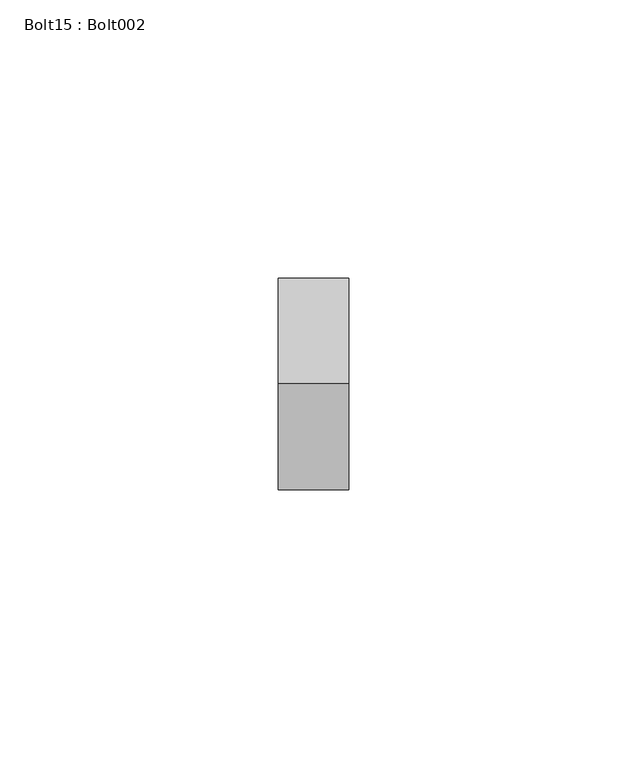
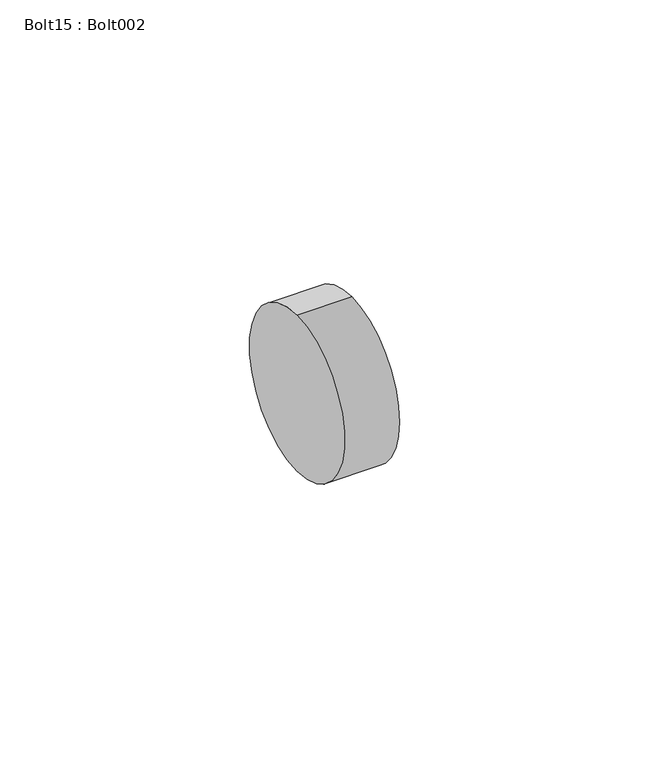
"""IFC4 building model written with IfcOpenShell, lengths in millimetres: proxy geometry, Bolt15 : Bolt002."""

import ifcopenshell
import ifcopenshell.guid

model = None  # the IFC model being written
_history = None  # IfcOwnerHistory: only IFC2X3 demands one
_inside = {}  # id of a spatial element -> (the spatial element, [elements in it])
_under = {}  # id of a project, library or spatial element -> (it, [spatial elements below it])
_declared = {}  # id of a project -> (the project, [libraries it declares])
_typed = {}  # id of a type object -> (the type object, [elements of that type])
_made_of = {}  # id of a material, layer set ... -> (it, [elements and type objects made of it])


def new_model(schema):
    """Start an empty IFC model of exactly this schema.

    Asked for "IFC4X3", IfcOpenShell would pick the latest addendum, in which some entities
    have other attributes; the version numbers below select the first issue.
    IFC2X3 requires an IfcOwnerHistory on every rooted entity: one is made here for all.
    """
    global model, _history
    if schema == "IFC4X3":
        model = ifcopenshell.file(schema_version=(4, 3, 0, 0))
    else:
        model = ifcopenshell.file(schema=schema)
    _inside.clear()
    _under.clear()
    _declared.clear()
    _typed.clear()
    _made_of.clear()
    _history = None
    if model.schema == "IFC2X3":
        org = make("IfcOrganization", Name="unknown")
        user = make(
            "IfcPersonAndOrganization",
            ThePerson=make("IfcPerson", FamilyName="unknown"),
            TheOrganization=org,
        )
        app = make(
            "IfcApplication",
            ApplicationDeveloper=org,
            Version="unknown",
            ApplicationFullName="unknown",
            ApplicationIdentifier="unknown",
        )
        _history = make(
            "IfcOwnerHistory",
            OwningUser=user,
            OwningApplication=app,
            ChangeAction="ADDED",
            CreationDate=0,
        )
    return model


def make(cls, **values):
    """One entity of the class cls with the attributes given. An attribute that is None is left unset."""
    return model.create_entity(
        cls, **{name: value for name, value in values.items() if value is not None}
    )


def rooted(cls, **values):
    """An entity with a GlobalId (a new one), such as an element, a storey or a relation."""
    return make(cls, GlobalId=ifcopenshell.guid.new(), OwnerHistory=_history, **values)


def si_unit(unit_type, name, prefix=None):
    """IfcSIUnit, for example si_unit("LENGTHUNIT", "METRE", prefix="MILLI")."""
    return make("IfcSIUnit", UnitType=unit_type, Prefix=prefix, Name=name)


def assignment(units):
    """IfcUnitAssignment: the units of a project."""
    return None if units is None else make("IfcUnitAssignment", Units=units)


def point(xyz):
    """IfcCartesianPoint."""
    return None if xyz is None else make("IfcCartesianPoint", Coordinates=xyz)


def direction(xyz):
    """IfcDirection."""
    return None if xyz is None else make("IfcDirection", DirectionRatios=xyz)


def frame(location, z_axis=None, x_axis=None):
    """IfcAxis2Placement3D, a coordinate frame: its origin and axes. An axis left out is left unset."""
    return make(
        "IfcAxis2Placement3D",
        Location=point(location),
        Axis=direction(z_axis),
        RefDirection=direction(x_axis),
    )


def frame_2d(location, x_axis=None):
    """IfcAxis2Placement2D, a coordinate frame in the plane: its origin and x axis."""
    return make(
        "IfcAxis2Placement2D", Location=point(location), RefDirection=direction(x_axis)
    )


def origin():
    """The frame at (0, 0, 0) with its axes left unset."""
    return frame((0.0, 0.0, 0.0))


def place(relative_to, where):
    """IfcLocalPlacement: puts the frame where relative to a parent placement (None: the world)."""
    return make(
        "IfcLocalPlacement", PlacementRelTo=relative_to, RelativePlacement=where
    )


def context(
    kind, dimensions, precision=None, world=None, true_north=None, identifier=None
):
    """IfcGeometricRepresentationContext, for example the 3D "Model" context."""
    return make(
        "IfcGeometricRepresentationContext",
        ContextIdentifier=identifier,
        ContextType=kind,
        CoordinateSpaceDimension=dimensions,
        Precision=precision,
        WorldCoordinateSystem=world,
        TrueNorth=true_north,
    )


def project(units=None, contexts=None):
    """IfcProject with its units and contexts."""
    return rooted(
        "IfcProject",
        Name="project",
        RepresentationContexts=contexts,
        UnitsInContext=assignment(units),
    )


def spatial(cls, under=None, at=None, **own):
    """A site, building, storey or space (cls), placed at a placement, below another one or the project."""
    s = rooted(cls, ObjectPlacement=at, **own)
    if under is not None:
        _under.setdefault(under.id(), (under, []))[1].append(s)
    return s


def circle_curve(where, radius):
    """IfcCircle in the frame where."""
    return make("IfcCircle", Position=where, Radius=radius)


def trimmed(basis, trim1, trim2, sense, master):
    """IfcTrimmedCurve: the piece of a basis curve between two trims."""
    return make(
        "IfcTrimmedCurve",
        BasisCurve=basis,
        Trim1=trim1,
        Trim2=trim2,
        SenseAgreement=sense,
        MasterRepresentation=master,
    )


def segment(curve, same_sense, transition):
    """IfcCompositeCurveSegment."""
    return make(
        "IfcCompositeCurveSegment",
        Transition=transition,
        SameSense=same_sense,
        ParentCurve=curve,
    )


def composite_curve(segments, self_intersect=None):
    """IfcCompositeCurve: segments joined end to end."""
    return make("IfcCompositeCurve", Segments=segments, SelfIntersect=self_intersect)


def outline(outer, holes=None, kind="AREA"):
    """IfcArbitraryClosedProfileDef: a profile drawn as a closed curve; with holes, ...WithVoids."""
    if holes is None:
        return make("IfcArbitraryClosedProfileDef", ProfileType=kind, OuterCurve=outer)
    return make(
        "IfcArbitraryProfileDefWithVoids",
        ProfileType=kind,
        OuterCurve=outer,
        InnerCurves=holes,
    )


def extrude(swept, where, along, depth):
    """IfcExtrudedAreaSolid: the profile swept, set in the frame where, extruded along a direction by depth."""
    return make(
        "IfcExtrudedAreaSolid",
        SweptArea=swept,
        Position=where,
        ExtrudedDirection=direction(along),
        Depth=depth,
    )


def shape(context_of_items, identifier, shape_type, items):
    """IfcShapeRepresentation: the items that make up one representation, for example the "Body"."""
    return make(
        "IfcShapeRepresentation",
        ContextOfItems=context_of_items,
        RepresentationIdentifier=identifier,
        RepresentationType=shape_type,
        Items=items,
    )


def source(mapping_origin, context_of_items, identifier, shape_type, items):
    """IfcRepresentationMap: a shape defined once, which mapped items show again and again."""
    return make(
        "IfcRepresentationMap",
        MappingOrigin=mapping_origin,
        MappedRepresentation=shape(context_of_items, identifier, shape_type, items),
    )


def transform(
    local_origin,
    x_axis=None,
    y_axis=None,
    z_axis=None,
    scale=None,
    scale2=None,
    scale3=None,
    uniform=True,
):
    """IfcCartesianTransformationOperator3D, or its non-uniform kind. x_axis, y_axis, z_axis: its Axis1, 2, 3."""
    if uniform:
        return make(
            "IfcCartesianTransformationOperator3D",
            Axis1=direction(x_axis),
            Axis2=direction(y_axis),
            LocalOrigin=point(local_origin),
            Scale=scale,
            Axis3=direction(z_axis),
        )
    return make(
        "IfcCartesianTransformationOperator3DnonUniform",
        Axis1=direction(x_axis),
        Axis2=direction(y_axis),
        LocalOrigin=point(local_origin),
        Scale=scale,
        Axis3=direction(z_axis),
        Scale2=scale2,
        Scale3=scale3,
    )


def mapped(mapping_source, mapping_target):
    """IfcMappedItem: shows the shape of a source again, moved by a transform."""
    return make(
        "IfcMappedItem", MappingSource=mapping_source, MappingTarget=mapping_target
    )


def made_of(thing, what):
    """Note that an element or type object is made of a material, layer set ...; save() writes the relation."""
    if what is not None:
        _made_of.setdefault(what.id(), (what, []))[1].append(thing)
    return thing


def element(
    cls,
    number,
    at=None,
    inside=None,
    cuts=None,
    type_object=None,
    material=None,
    context=None,
    identifier="Body",
    shape_type=None,
    held_by="IfcProductDefinitionShape",
    body=None,
    shapes=None,
    **own,
):
    """One element of the class cls, such as IfcWall. Its Tag is "e" and its number.

    at: its placement. inside: the storey or other place that contains it. cuts: it is an
    opening in that element (IfcRelVoidsElement). A single representation is given by context,
    identifier, shape_type and body (its items); several are given by shapes. held_by: the class
    of the entity that holds the representations. save() writes the other relations.
    """
    e = rooted(cls, Tag="e%d" % number, ObjectPlacement=at, **own)
    if body is not None:
        shapes = [shape(context, identifier, shape_type, body)]
    if shapes is not None:
        e.Representation = make(held_by, Representations=shapes)
    if inside is not None:
        _inside.setdefault(inside.id(), (inside, []))[1].append(e)
    if cuts is not None:
        rooted(
            "IfcRelVoidsElement", RelatingBuildingElement=cuts, RelatedOpeningElement=e
        )
    if type_object is not None:
        _typed.setdefault(type_object.id(), (type_object, []))[1].append(e)
    return made_of(e, material)


def aggregate(whole, parts):
    """IfcRelAggregates: a whole, such as a stair, and the parts it consists of."""
    return rooted("IfcRelAggregates", RelatingObject=whole, RelatedObjects=parts)


def save(model, path):
    """Write the relations noted so far, then the file.

    IfcRelAggregates (storeys below a building ...), IfcRelContainedInSpatialStructure (elements
    in a storey), IfcRelDefinesByType, IfcRelAssociatesMaterial and IfcRelDeclares: one each for
    every whole, place, type object, material and project.
    """
    for whole, parts in _under.values():
        aggregate(whole, parts)
    for where, things in _inside.values():
        rooted(
            "IfcRelContainedInSpatialStructure",
            RelatedElements=things,
            RelatingStructure=where,
        )
    for kind, things in _typed.values():
        rooted("IfcRelDefinesByType", RelatedObjects=things, RelatingType=kind)
    for what, things in _made_of.values():
        rooted("IfcRelAssociatesMaterial", RelatedObjects=things, RelatingMaterial=what)
    for by, libraries in _declared.values():
        rooted("IfcRelDeclares", RelatingContext=by, RelatedDefinitions=libraries)
    model.write(path)


def bolt15_bolt002_170dc097(model_context):
    return source(origin(), model_context, "Body", "SweptSolid", [
        extrude(outline(composite_curve([segment(trimmed(circle_curve(frame_2d((1896.5882072, 39910.0063132)), 19.05), [point((1896.5882072, 39929.0563132))], [point((1896.5882072, 39890.9563132))], False, "CARTESIAN"), True, "CONTINUOUS"), segment(trimmed(circle_curve(frame_2d((1896.5882072, 39910.0063132)), 19.05), [point((1896.5882072, 39890.9563132))], [point((1896.5882072, 39929.0563132))], False, "CARTESIAN"), True, "CONTINUOUS")], self_intersect=False)), frame((10297.8384869, 0.0, 0.0), z_axis=(1.0, 0.0, 0.0), x_axis=(0.0, 1.0, 0.0)), (0.0, 0.0, 1.0), 12.7),
    ])


if __name__ == "__main__":
    model = new_model("IFC4")
    model_context = context("Model", 3, world=origin())
    ifc_project = project(units=[si_unit("LENGTHUNIT", "METRE", prefix="MILLI")], contexts=[model_context])
    site = spatial("IfcSite", under=ifc_project)
    building = spatial("IfcBuilding", under=site)
    placement = place(None, origin())
    bolt15_bolt002_shape = bolt15_bolt002_170dc097(model_context)
    element("IfcBuildingElementProxy", 1, Name="Bolt15 : Bolt002", ObjectType="Bolt15 : Bolt002", at=placement, inside=building, context=model_context, shape_type="MappedRepresentation", body=[
        mapped(bolt15_bolt002_shape, transform((0.0, 0.0, 0.0), x_axis=(1.0, 0.0, 0.0), y_axis=(0.0, 1.0, 0.0), z_axis=(0.0, 0.0, 1.0))),
    ])
    save(model, "model.ifc")

# Revit data of these elements
# Type "Bolt15 : Bolt002"
#   NameOverride = "Bolt002"
# Element 1 (IfcBuildingElementProxy, "Bolt15 : Bolt002")
#   Materials on its faces: "TUBE STEEL STRINGER WELDED TO ANCHORED STEEL PLATE - SEE STRUCT DWGS"
# Materials
#   "TUBE STEEL STRINGER WELDED TO ANCHORED STEEL PLATE - SEE STRUCT DWGS": class "Unassigned", colour RGB 128 128 128, transparency 0, Cost = 0
